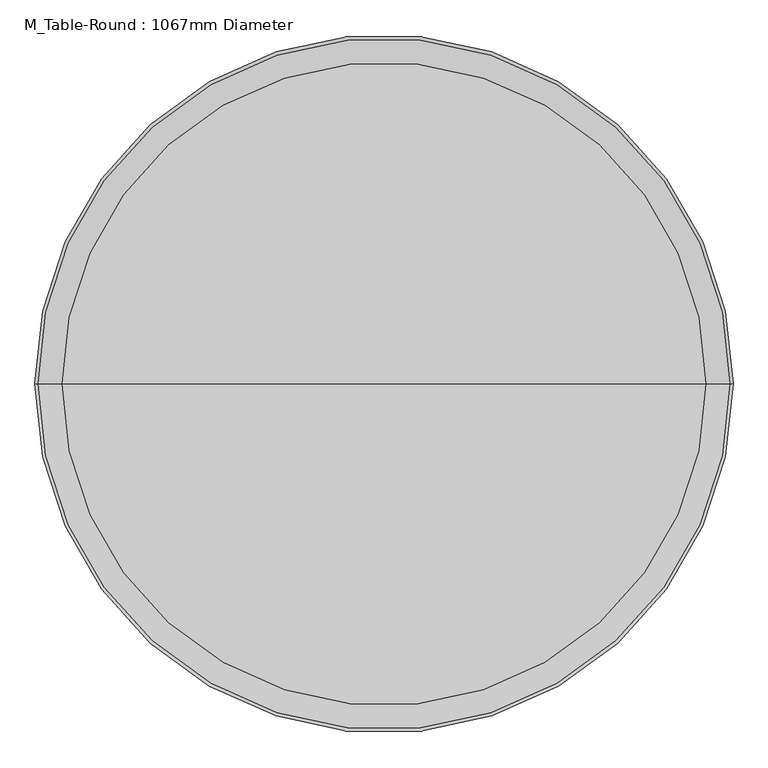
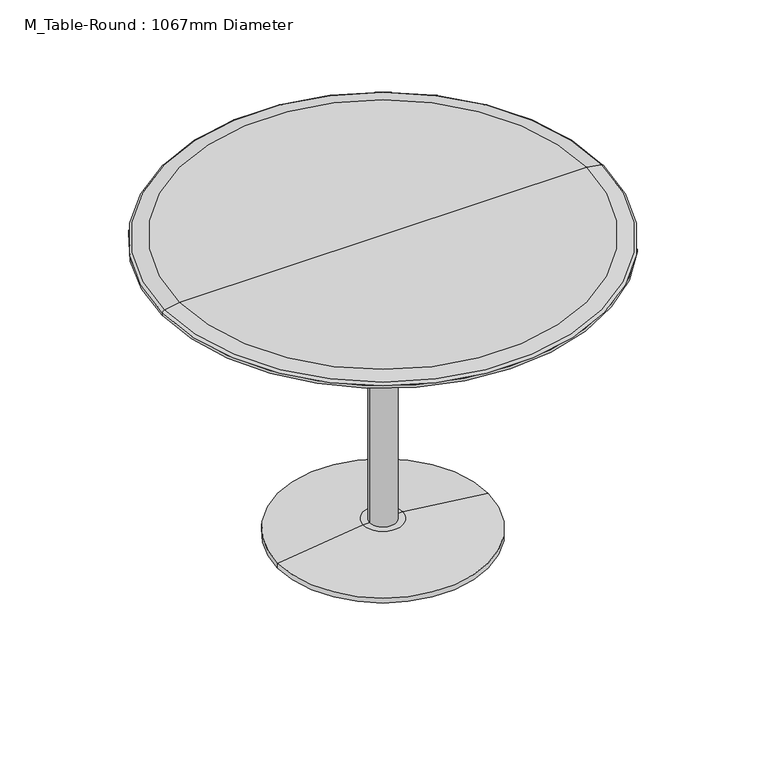
"""IFC4 building model written with IfcOpenShell, lengths in millimetres: furniture geometry, M_Table-Round : 1067mm Diameter."""

from ifc_helpers import new_model, si_unit, point, frame, origin, origin_2d, place, context, project, spatial, polyline, circle_curve, ellipse_curve, trimmed, segment, composite_curve, outline, extrude, source, transform, mapped, element, save
from ifc_brep_helpers import plane_surface, cylinder_surface, revolved_surface, advanced_brep


def m_table_round_1067mm_diameter_968811aa(model_context):
    return source(origin(), model_context, "Body", "SolidModel", [
        extrude(outline(composite_curve([segment(trimmed(circle_curve(origin_2d(), 31.75), [point((-31.75, 0.0))], [point((31.75, 0.0))], False, "CARTESIAN"), True, "CONTINUOUS"), segment(trimmed(circle_curve(origin_2d(), 31.75), [point((31.75, 0.0))], [point((-31.75, 0.0))], False, "CARTESIAN"), True, "CONTINUOUS")], self_intersect=False)), frame((0.0, 0.0, 38.1), z_axis=(0.0, 0.0, 1.0), x_axis=(1.0, 0.0, 0.0)), (0.0, 0.0, 1.0), 704.85),
        advanced_brep(
        [(0.0, 0.0, 742.95), (-533.0, 0.0, 742.95), (533.0, 0.0, 742.95), (491.1011364, 0.0, 762.0), (-491.1011364, 0.0, 762.0), (0.0, 0.0, 762.0), (527.7526659, 0.0, 755.5373465), (-527.7526659, 0.0, 755.5373465), (533.0, 0.0, 749.2838172), (-533.0, 0.0, 749.2838172)],
        [
            (0, 1),
            (1, 2, circle_curve(frame((0.0, 0.0, 742.95), z_axis=(0.0, 0.0, -1.0), x_axis=(-1.0, 0.0, 0.0)), 533.0)),
            (2, 0),
            (2, 1, circle_curve(frame((0.0, 0.0, 742.95), z_axis=(0.0, 0.0, -1.0), x_axis=(-1.0, 0.0, 0.0)), 533.0)),
            (3, 4, circle_curve(frame((0.0, 0.0, 762.0), z_axis=(0.0, 0.0, 1.0), x_axis=(-1.0, 0.0, 0.0)), 491.1011364)),
            (4, 5),
            (5, 3),
            (4, 3, circle_curve(frame((0.0, 0.0, 762.0), z_axis=(0.0, 0.0, 1.0), x_axis=(-1.0, 0.0, 0.0)), 491.1011364)),
            (6, 7, circle_curve(frame((0.0, 0.0, 755.5373465), z_axis=(0.0, 0.0, 1.0), x_axis=(-1.0, 0.0, 0.0)), 527.7526659)),
            (7, 4),
            (3, 6),
            (7, 6, circle_curve(frame((0.0, 0.0, 755.5373465), z_axis=(0.0, 0.0, 1.0), x_axis=(-1.0, 0.0, 0.0)), 527.7526659)),
            (8, 9, circle_curve(frame((0.0, 0.0, 749.2838172), z_axis=(0.0, 0.0, 1.0), x_axis=(-1.0, 0.0, 0.0)), 533.0)),
            (9, 7, circle_curve(frame((-526.65, 0.0, 749.2838172), z_axis=(0.0, 1.0, 0.0), x_axis=(1.0, 0.0, 0.0)), 6.35)),
            (6, 8, circle_curve(frame((526.65, 0.0, 749.2838172), z_axis=(0.0, 1.0, 0.0), x_axis=(-1.0, 0.0, 0.0)), 6.35)),
            (9, 8, circle_curve(frame((0.0, 0.0, 749.2838172), z_axis=(0.0, 0.0, 1.0), x_axis=(-1.0, 0.0, 0.0)), 533.0)),
            (1, 9),
            (8, 2),
        ],
        [
            plane_surface(frame((0.0, 0.0, 742.95), z_axis=(0.0, 0.0, -1.0), x_axis=(-1.0, 0.0, 0.0))),
            plane_surface(frame((0.0, 0.0, 762.0), z_axis=(0.0, 0.0, 1.0), x_axis=(-1.0, 0.0, 0.0))),
            revolved_surface(polyline([(-491.1011364, 0.0, 762.0), (-527.7526659, 0.0, 755.5373465)]), (0.0, 0.0, 838.2), (0.0, 0.0, -1.0)),
            revolved_surface(trimmed(ellipse_curve(frame((-526.65, 0.0, 749.2838172), z_axis=(0.0, -1.0, 0.0), x_axis=(1.0, 0.0, 0.0)), 6.35, 6.35), [point((-527.7526659, 0.0, 755.5373465))], [point((-533.0, 0.0, 749.2838172))], True, "CARTESIAN"), (0.0, 0.0, 838.2), (0.0, 0.0, -1.0)),
            cylinder_surface(frame((0.0, 0.0, 838.2), z_axis=(0.0, 0.0, -1.0), x_axis=(-1.0, 0.0, 0.0)), 533.0),
        ],
        [
            (0, [[1, 2, 3]]),
            (0, [[-3, 4, -1]]),
            (1, [[5, 6, 7]]),
            (1, [[8, -7, -6]]),
            (2, [[9, 10, -5, 11]]),
            (2, [[12, -11, -8, -10]]),
            (3, [[13, 14, -9, 15]]),
            (3, [[16, -15, -12, -14]]),
            (4, [[-2, 17, -13, 18]]),
            (4, [[-4, -18, -16, -17]]),
        ],
    ),
        advanced_brep(
        [(0.0, 0.0, 0.0), (-254.0, 0.0, 0.0), (254.0, 0.0, 0.0), (47.625, 0.0, 38.1), (-47.625, 0.0, 38.1), (0.0, 0.0, 38.1), (254.0, 0.0, 12.7), (-254.0, 0.0, 12.7)],
        [
            (0, 1),
            (1, 2, circle_curve(frame((0.0, 0.0, 0.0), z_axis=(0.0, 0.0, -1.0), x_axis=(-1.0, 0.0, 0.0)), 254.0)),
            (2, 0),
            (2, 1, circle_curve(frame((0.0, 0.0, 0.0), z_axis=(0.0, 0.0, -1.0), x_axis=(-1.0, 0.0, 0.0)), 254.0)),
            (3, 4, circle_curve(frame((0.0, 0.0, 38.1), z_axis=(0.0, 0.0, 1.0), x_axis=(-1.0, 0.0, 0.0)), 47.625)),
            (4, 5),
            (5, 3),
            (4, 3, circle_curve(frame((0.0, 0.0, 38.1), z_axis=(0.0, 0.0, 1.0), x_axis=(-1.0, 0.0, 0.0)), 47.625)),
            (6, 7, circle_curve(frame((0.0, 0.0, 12.7), z_axis=(0.0, 0.0, 1.0), x_axis=(-1.0, 0.0, 0.0)), 254.0)),
            (7, 4),
            (3, 6),
            (7, 6, circle_curve(frame((0.0, 0.0, 12.7), z_axis=(0.0, 0.0, 1.0), x_axis=(-1.0, 0.0, 0.0)), 254.0)),
            (1, 7),
            (6, 2),
        ],
        [
            plane_surface(frame((0.0, 0.0, 0.0), z_axis=(0.0, 0.0, -1.0), x_axis=(-1.0, 0.0, 0.0))),
            plane_surface(frame((0.0, 0.0, 38.1), z_axis=(0.0, 0.0, 1.0), x_axis=(-1.0, 0.0, 0.0))),
            revolved_surface(polyline([(-47.625, 0.0, 38.1), (-254.0, 0.0, 12.7)]), (0.0, 0.0, 215.9), (0.0, 0.0, -1.0)),
            cylinder_surface(frame((0.0, 0.0, 215.9), z_axis=(0.0, 0.0, -1.0), x_axis=(-1.0, 0.0, 0.0)), 254.0),
        ],
        [
            (0, [[1, 2, 3]]),
            (0, [[-3, 4, -1]]),
            (1, [[5, 6, 7]]),
            (1, [[8, -7, -6]]),
            (2, [[9, 10, -5, 11]]),
            (2, [[12, -11, -8, -10]]),
            (3, [[-2, 13, -9, 14]]),
            (3, [[-4, -14, -12, -13]]),
        ],
    ),
    ])


if __name__ == "__main__":
    model = new_model("IFC4")
    model_context = context("Model", 3, world=origin())
    ifc_project = project(units=[si_unit("LENGTHUNIT", "METRE", prefix="MILLI")], contexts=[model_context])
    site = spatial("IfcSite", under=ifc_project)
    building = spatial("IfcBuilding", under=site)
    placement = place(None, origin())
    m_table_round_1067mm_diameter_shape = m_table_round_1067mm_diameter_968811aa(model_context)
    element("IfcFurniture", 1, ObjectType="M_Table-Round : 1067mm Diameter", at=placement, inside=building, context=model_context, shape_type="MappedRepresentation", body=[
        mapped(m_table_round_1067mm_diameter_shape, transform((0.0, 0.0, 0.0), x_axis=(1.0, 0.0, 0.0), y_axis=(0.0, 1.0, 0.0), z_axis=(0.0, 0.0, 1.0))),
    ])
    save(model, "model.ifc")

# Revit data of these elements
# Type "M_Table-Round : 1067mm Diameter"
#   Base Radius = 0.254 m
#   Height = 0.762 m
#   Radius = 0.533 m
#   Base Material = Steel, Chrome Plated
#   Top Material = Birch
# Element 1 (IfcFurniture, "M_Table-Round : 1067mm Diameter")
#   Materials on its faces: "Steel, Chrome Plated", "Birch"
# Materials
#   "Steel, Chrome Plated": class "Metal", colour RGB 244 244 244, transparency 0, Description = "Chromiuim plated steel", Cost = 0
#   "Birch": class "Wood", colour RGB 224 178 126, transparency 0, Description = "Betula Alleghaniensis", Cost = 0
